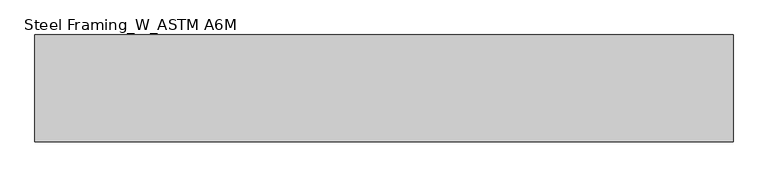
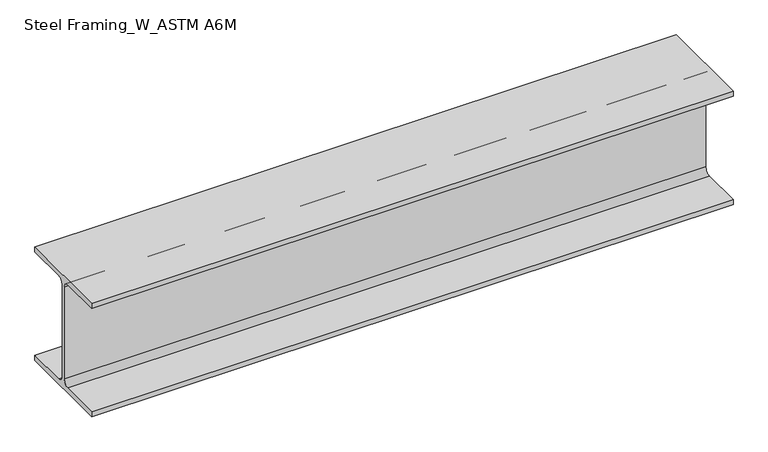
"""IFC4 building model written with IfcOpenShell, lengths in millimetres: beam geometry, Steel Framing_W_ASTM A6M : H_SB_AR_S02_W250x49.1_G5."""

import ifcopenshell
import ifcopenshell.guid

model = None  # the IFC model being written
_history = None  # IfcOwnerHistory: only IFC2X3 demands one
_inside = {}  # id of a spatial element -> (the spatial element, [elements in it])
_under = {}  # id of a project, library or spatial element -> (it, [spatial elements below it])
_declared = {}  # id of a project -> (the project, [libraries it declares])
_typed = {}  # id of a type object -> (the type object, [elements of that type])
_made_of = {}  # id of a material, layer set ... -> (it, [elements and type objects made of it])


def new_model(schema):
    """Start an empty IFC model of exactly this schema.

    Asked for "IFC4X3", IfcOpenShell would pick the latest addendum, in which some entities
    have other attributes; the version numbers below select the first issue.
    IFC2X3 requires an IfcOwnerHistory on every rooted entity: one is made here for all.
    """
    global model, _history
    if schema == "IFC4X3":
        model = ifcopenshell.file(schema_version=(4, 3, 0, 0))
    else:
        model = ifcopenshell.file(schema=schema)
    _inside.clear()
    _under.clear()
    _declared.clear()
    _typed.clear()
    _made_of.clear()
    _history = None
    if model.schema == "IFC2X3":
        org = make("IfcOrganization", Name="unknown")
        user = make(
            "IfcPersonAndOrganization",
            ThePerson=make("IfcPerson", FamilyName="unknown"),
            TheOrganization=org,
        )
        app = make(
            "IfcApplication",
            ApplicationDeveloper=org,
            Version="unknown",
            ApplicationFullName="unknown",
            ApplicationIdentifier="unknown",
        )
        _history = make(
            "IfcOwnerHistory",
            OwningUser=user,
            OwningApplication=app,
            ChangeAction="ADDED",
            CreationDate=0,
        )
    return model


def make(cls, **values):
    """One entity of the class cls with the attributes given. An attribute that is None is left unset."""
    return model.create_entity(
        cls, **{name: value for name, value in values.items() if value is not None}
    )


def rooted(cls, **values):
    """An entity with a GlobalId (a new one), such as an element, a storey or a relation."""
    return make(cls, GlobalId=ifcopenshell.guid.new(), OwnerHistory=_history, **values)


def si_unit(unit_type, name, prefix=None):
    """IfcSIUnit, for example si_unit("LENGTHUNIT", "METRE", prefix="MILLI")."""
    return make("IfcSIUnit", UnitType=unit_type, Prefix=prefix, Name=name)


def assignment(units):
    """IfcUnitAssignment: the units of a project."""
    return None if units is None else make("IfcUnitAssignment", Units=units)


def point(xyz):
    """IfcCartesianPoint."""
    return None if xyz is None else make("IfcCartesianPoint", Coordinates=xyz)


def direction(xyz):
    """IfcDirection."""
    return None if xyz is None else make("IfcDirection", DirectionRatios=xyz)


def frame(location, z_axis=None, x_axis=None):
    """IfcAxis2Placement3D, a coordinate frame: its origin and axes. An axis left out is left unset."""
    return make(
        "IfcAxis2Placement3D",
        Location=point(location),
        Axis=direction(z_axis),
        RefDirection=direction(x_axis),
    )


def frame_2d(location, x_axis=None):
    """IfcAxis2Placement2D, a coordinate frame in the plane: its origin and x axis."""
    return make(
        "IfcAxis2Placement2D", Location=point(location), RefDirection=direction(x_axis)
    )


def origin():
    """The frame at (0, 0, 0) with its axes left unset."""
    return frame((0.0, 0.0, 0.0))


def place(relative_to, where):
    """IfcLocalPlacement: puts the frame where relative to a parent placement (None: the world)."""
    return make(
        "IfcLocalPlacement", PlacementRelTo=relative_to, RelativePlacement=where
    )


def context(
    kind, dimensions, precision=None, world=None, true_north=None, identifier=None
):
    """IfcGeometricRepresentationContext, for example the 3D "Model" context."""
    return make(
        "IfcGeometricRepresentationContext",
        ContextIdentifier=identifier,
        ContextType=kind,
        CoordinateSpaceDimension=dimensions,
        Precision=precision,
        WorldCoordinateSystem=world,
        TrueNorth=true_north,
    )


def project(units=None, contexts=None):
    """IfcProject with its units and contexts."""
    return rooted(
        "IfcProject",
        Name="project",
        RepresentationContexts=contexts,
        UnitsInContext=assignment(units),
    )


def spatial(cls, under=None, at=None, **own):
    """A site, building, storey or space (cls), placed at a placement, below another one or the project."""
    s = rooted(cls, ObjectPlacement=at, **own)
    if under is not None:
        _under.setdefault(under.id(), (under, []))[1].append(s)
    return s


def polyline(points):
    """IfcPolyline through the points."""
    return make("IfcPolyline", Points=[point(p) for p in points])


def circle_curve(where, radius):
    """IfcCircle in the frame where."""
    return make("IfcCircle", Position=where, Radius=radius)


def trimmed(basis, trim1, trim2, sense, master):
    """IfcTrimmedCurve: the piece of a basis curve between two trims."""
    return make(
        "IfcTrimmedCurve",
        BasisCurve=basis,
        Trim1=trim1,
        Trim2=trim2,
        SenseAgreement=sense,
        MasterRepresentation=master,
    )


def segment(curve, same_sense, transition):
    """IfcCompositeCurveSegment."""
    return make(
        "IfcCompositeCurveSegment",
        Transition=transition,
        SameSense=same_sense,
        ParentCurve=curve,
    )


def composite_curve(segments, self_intersect=None):
    """IfcCompositeCurve: segments joined end to end."""
    return make("IfcCompositeCurve", Segments=segments, SelfIntersect=self_intersect)


def outline(outer, holes=None, kind="AREA"):
    """IfcArbitraryClosedProfileDef: a profile drawn as a closed curve; with holes, ...WithVoids."""
    if holes is None:
        return make("IfcArbitraryClosedProfileDef", ProfileType=kind, OuterCurve=outer)
    return make(
        "IfcArbitraryProfileDefWithVoids",
        ProfileType=kind,
        OuterCurve=outer,
        InnerCurves=holes,
    )


def extrude(swept, where, along, depth):
    """IfcExtrudedAreaSolid: the profile swept, set in the frame where, extruded along a direction by depth."""
    return make(
        "IfcExtrudedAreaSolid",
        SweptArea=swept,
        Position=where,
        ExtrudedDirection=direction(along),
        Depth=depth,
    )


def shape(context_of_items, identifier, shape_type, items):
    """IfcShapeRepresentation: the items that make up one representation, for example the "Body"."""
    return make(
        "IfcShapeRepresentation",
        ContextOfItems=context_of_items,
        RepresentationIdentifier=identifier,
        RepresentationType=shape_type,
        Items=items,
    )


def source(mapping_origin, context_of_items, identifier, shape_type, items):
    """IfcRepresentationMap: a shape defined once, which mapped items show again and again."""
    return make(
        "IfcRepresentationMap",
        MappingOrigin=mapping_origin,
        MappedRepresentation=shape(context_of_items, identifier, shape_type, items),
    )


def transform(
    local_origin,
    x_axis=None,
    y_axis=None,
    z_axis=None,
    scale=None,
    scale2=None,
    scale3=None,
    uniform=True,
):
    """IfcCartesianTransformationOperator3D, or its non-uniform kind. x_axis, y_axis, z_axis: its Axis1, 2, 3."""
    if uniform:
        return make(
            "IfcCartesianTransformationOperator3D",
            Axis1=direction(x_axis),
            Axis2=direction(y_axis),
            LocalOrigin=point(local_origin),
            Scale=scale,
            Axis3=direction(z_axis),
        )
    return make(
        "IfcCartesianTransformationOperator3DnonUniform",
        Axis1=direction(x_axis),
        Axis2=direction(y_axis),
        LocalOrigin=point(local_origin),
        Scale=scale,
        Axis3=direction(z_axis),
        Scale2=scale2,
        Scale3=scale3,
    )


def mapped(mapping_source, mapping_target):
    """IfcMappedItem: shows the shape of a source again, moved by a transform."""
    return make(
        "IfcMappedItem", MappingSource=mapping_source, MappingTarget=mapping_target
    )


def made_of(thing, what):
    """Note that an element or type object is made of a material, layer set ...; save() writes the relation."""
    if what is not None:
        _made_of.setdefault(what.id(), (what, []))[1].append(thing)
    return thing


def element(
    cls,
    number,
    at=None,
    inside=None,
    cuts=None,
    type_object=None,
    material=None,
    context=None,
    identifier="Body",
    shape_type=None,
    held_by="IfcProductDefinitionShape",
    body=None,
    shapes=None,
    **own,
):
    """One element of the class cls, such as IfcWall. Its Tag is "e" and its number.

    at: its placement. inside: the storey or other place that contains it. cuts: it is an
    opening in that element (IfcRelVoidsElement). A single representation is given by context,
    identifier, shape_type and body (its items); several are given by shapes. held_by: the class
    of the entity that holds the representations. save() writes the other relations.
    """
    e = rooted(cls, Tag="e%d" % number, ObjectPlacement=at, **own)
    if body is not None:
        shapes = [shape(context, identifier, shape_type, body)]
    if shapes is not None:
        e.Representation = make(held_by, Representations=shapes)
    if inside is not None:
        _inside.setdefault(inside.id(), (inside, []))[1].append(e)
    if cuts is not None:
        rooted(
            "IfcRelVoidsElement", RelatingBuildingElement=cuts, RelatedOpeningElement=e
        )
    if type_object is not None:
        _typed.setdefault(type_object.id(), (type_object, []))[1].append(e)
    return made_of(e, material)


def aggregate(whole, parts):
    """IfcRelAggregates: a whole, such as a stair, and the parts it consists of."""
    return rooted("IfcRelAggregates", RelatingObject=whole, RelatedObjects=parts)


def save(model, path):
    """Write the relations noted so far, then the file.

    IfcRelAggregates (storeys below a building ...), IfcRelContainedInSpatialStructure (elements
    in a storey), IfcRelDefinesByType, IfcRelAssociatesMaterial and IfcRelDeclares: one each for
    every whole, place, type object, material and project.
    """
    for whole, parts in _under.values():
        aggregate(whole, parts)
    for where, things in _inside.values():
        rooted(
            "IfcRelContainedInSpatialStructure",
            RelatedElements=things,
            RelatingStructure=where,
        )
    for kind, things in _typed.values():
        rooted("IfcRelDefinesByType", RelatedObjects=things, RelatingType=kind)
    for what, things in _made_of.values():
        rooted("IfcRelAssociatesMaterial", RelatedObjects=things, RelatingMaterial=what)
    for by, libraries in _declared.values():
        rooted("IfcRelDeclares", RelatingContext=by, RelatedDefinitions=libraries)
    model.write(path)


def steel_framing_w_astm_a6m_7f0d9279(model_context):
    return source(origin(), model_context, "Body", "SweptSolid", [
        extrude(outline(composite_curve([segment(polyline([(101.0, -112.5), (101.0, -123.5), (-101.0, -123.5), (-101.0, -112.5), (-16.385, -112.5)]), True, "CONTINUOUS"), segment(trimmed(circle_curve(frame_2d((-16.385, -99.8)), 12.7), [point((-16.385, -112.5))], [point((-3.685, -99.8))], True, "CARTESIAN"), True, "CONTINUOUS"), segment(polyline([(-3.685, -99.8), (-3.685, 99.8)]), True, "CONTINUOUS"), segment(trimmed(circle_curve(frame_2d((-16.385, 99.8)), 12.7), [point((-3.685, 99.8))], [point((-16.385, 112.5))], True, "CARTESIAN"), True, "CONTINUOUS"), segment(polyline([(-16.385, 112.5), (-101.0, 112.5), (-101.0, 123.5), (101.0, 123.5), (101.0, 112.5), (16.385, 112.5)]), True, "CONTINUOUS"), segment(trimmed(circle_curve(frame_2d((16.385, 99.8)), 12.7), [point((16.385, 112.5))], [point((3.685, 99.8))], True, "CARTESIAN"), True, "CONTINUOUS"), segment(polyline([(3.685, 99.8), (3.685, -99.8)]), True, "CONTINUOUS"), segment(trimmed(circle_curve(frame_2d((16.385, -99.8)), 12.7), [point((3.685, -99.8))], [point((16.385, -112.5))], True, "CARTESIAN"), True, "CONTINUOUS"), segment(polyline([(16.385, -112.5), (101.0, -112.5)]), True, "CONTINUOUS")], self_intersect=False)), frame((-503.8, 0.0, 0.0), z_axis=(1.0, 0.0, 0.0), x_axis=(0.0, 1.0, 0.0)), (0.0, 0.0, 1.0), 1320.8),
    ])


if __name__ == "__main__":
    model = new_model("IFC4")
    model_context = context("Model", 3, world=origin())
    ifc_project = project(units=[si_unit("LENGTHUNIT", "METRE", prefix="MILLI")], contexts=[model_context])
    site = spatial("IfcSite", under=ifc_project)
    building = spatial("IfcBuilding", under=site)
    placement = place(None, origin())
    steel_framing_w_astm_a6m_shape = steel_framing_w_astm_a6m_7f0d9279(model_context)
    element("IfcBeam", 1, ObjectType="Steel Framing_W_ASTM A6M : H_SB_AR_S02_W250x49.1_G5", at=placement, inside=building, context=model_context, shape_type="MappedRepresentation", body=[
        mapped(steel_framing_w_astm_a6m_shape, transform((0.0, 0.0, 0.0), x_axis=(1.0, 0.0, 0.0), y_axis=(0.0, 1.0, 0.0), z_axis=(0.0, 0.0, 1.0))),
    ])
    save(model, "model.ifc")

# Revit data of these elements
# Type "Steel Framing_W_ASTM A6M : H_SB_AR_S02_W250x49.1_G5"
#   Type Mark = "G5"
#   Section Name Key = "W10x33"
#   Width = 20.2 cm
#   Web Thickness = 0.737 cm
#   Web Fillet = 1.27 cm
#   Warping Constant = 212000.0 cm⁶
#   Torsional Moment of Inertia = 24.30 cm⁴
#   Section Area = 62.6 cm²
#   Plastic Modulus weak axis = 229.0 cm³
#   Plastic Modulus strong axis = 636.0 cm³
#   Perimeter = 1.27 m²/m
#   Nominal Weight = 49.10 kgf/m
#   Moment of Inertia weak axis = 1520.00 cm⁴
#   Moment of Inertia strong axis = 7120.00 cm⁴
#   Height = 24.7 cm
#   Flange Thickness = 1.1 cm
#   Elastic Modulus weak axis = 151.0 cm³
#   Elastic Modulus strong axis = 574.0 cm³
#   Centroid Vertical = 12.35 cm
#   Centroid Horizontal = 10.1 cm
#   Length [instance default] = 1500 mm
#   Structural Material [instance default] = Steel, 45-345
#   Bolt Spacing = 0
#   Assembly Code = ""
# Element 1 (IfcBeam, "Steel Framing_W_ASTM A6M : H_SB_AR_S02_W250x49.1_G5")
#   Materials on its faces: "Steel, 45-345"
# Materials
#   "Steel, 45-345": class "Metal", colour RGB 189 187 185, transparency 0, Description = "Steel 345 MPa", Cost = 0
